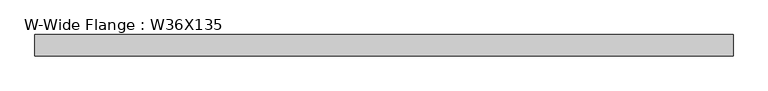
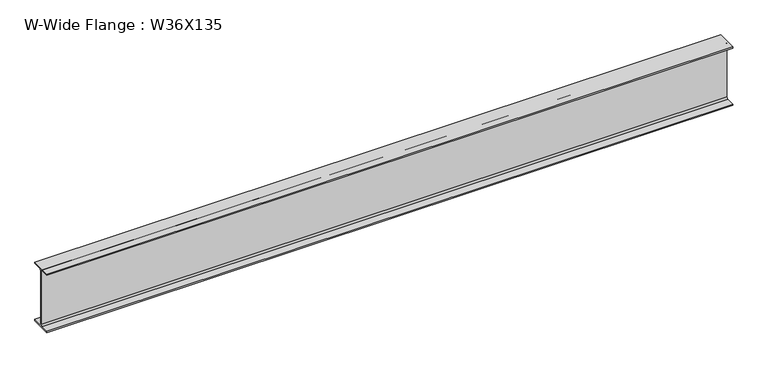
"""IFC4 building model written with IfcOpenShell, lengths in millimetres: beam geometry, W-Wide Flange : W36X135."""

from ifc_helpers import new_model, si_unit, point, frame, frame_2d, origin, place, context, project, spatial, polyline, circle_curve, trimmed, segment, composite_curve, outline, extrude, source, transform, mapped, element, save


def w_wide_flange_w36x135_915bd06f(model_context):
    return source(origin(), model_context, "Body", "SweptSolid", [
        extrude(outline(composite_curve([segment(polyline([(152.4, -432.054), (152.4, -452.12), (-152.4, -452.12), (-152.4, -432.054), (-30.4165, -432.054)]), True, "CONTINUOUS"), segment(trimmed(circle_curve(frame_2d((-30.4165, -409.2575)), 22.7965), [point((-30.4165, -432.054))], [point((-7.62, -409.2575))], True, "CARTESIAN"), True, "CONTINUOUS"), segment(polyline([(-7.62, -409.2575), (-7.62, 409.2575)]), True, "CONTINUOUS"), segment(trimmed(circle_curve(frame_2d((-30.4165, 409.2575)), 22.7965), [point((-7.62, 409.2575))], [point((-30.4165, 432.054))], True, "CARTESIAN"), True, "CONTINUOUS"), segment(polyline([(-30.4165, 432.054), (-152.4, 432.054), (-152.4, 452.12), (152.4, 452.12), (152.4, 432.054), (30.4165, 432.054)]), True, "CONTINUOUS"), segment(trimmed(circle_curve(frame_2d((30.4165, 409.2575)), 22.7965), [point((30.4165, 432.054))], [point((7.62, 409.2575))], True, "CARTESIAN"), True, "CONTINUOUS"), segment(polyline([(7.62, 409.2575), (7.62, -409.2575)]), True, "CONTINUOUS"), segment(trimmed(circle_curve(frame_2d((30.4165, -409.2575)), 22.7965), [point((7.62, -409.2575))], [point((30.4165, -432.054))], True, "CARTESIAN"), True, "CONTINUOUS"), segment(polyline([(30.4165, -432.054), (152.4, -432.054)]), True, "CONTINUOUS")], self_intersect=False)), frame((-4965.3459352, 0.0, 0.0), z_axis=(1.0, 0.0, 0.0), x_axis=(0.0, 1.0, 0.0)), (0.0, 0.0, 1.0), 10026.09201),
    ])


if __name__ == "__main__":
    model = new_model("IFC4")
    model_context = context("Model", 3, world=origin())
    ifc_project = project(units=[si_unit("LENGTHUNIT", "METRE", prefix="MILLI")], contexts=[model_context])
    site = spatial("IfcSite", under=ifc_project)
    building = spatial("IfcBuilding", under=site)
    placement = place(None, origin())
    w_wide_flange_w36x135_shape = w_wide_flange_w36x135_915bd06f(model_context)
    element("IfcBeam", 1, ObjectType="W-Wide Flange : W36X135", at=placement, inside=building, context=model_context, shape_type="MappedRepresentation", body=[
        mapped(w_wide_flange_w36x135_shape, transform((0.0, 0.0, 0.0), x_axis=(1.0, 0.0, 0.0), y_axis=(0.0, 1.0, 0.0), z_axis=(0.0, 0.0, 1.0))),
    ])
    save(model, "model.ifc")

# Revit data of these elements
# Type "W-Wide Flange : W36X135"
#   Assembly Code = "B10"
#   W = 135
#   Length [instance default] = 1524 mm
#   bf = 304.8 mm
#   d = 904.24 mm
#   k = 42.863 mm
#   k2 = 22.797 mm
#   tf = 20.066 mm
#   tw = 15.24 mm
#   A = 0.0256129 m²
#   Structural Material [instance default] = Steel ASTM A992
# Element 1 (IfcBeam, "W-Wide Flange : W36X135")
#   Structural Material = Aluminum, Anodized Red
#   Materials on its faces: "Aluminum, Anodized Red"
# Materials
#   "Steel ASTM A992": class "Metal", colour RGB 128 0 0, transparency 0, Description = "Structural steel 50ksi", Cost = 0
#   "Aluminum, Anodized Red": class "Metal", colour RGB 120 120 120, transparency 0, Description = "Anodized aluminum, red", Cost = 0
